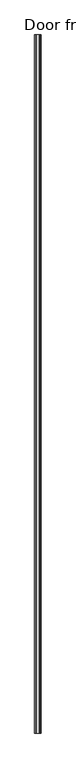
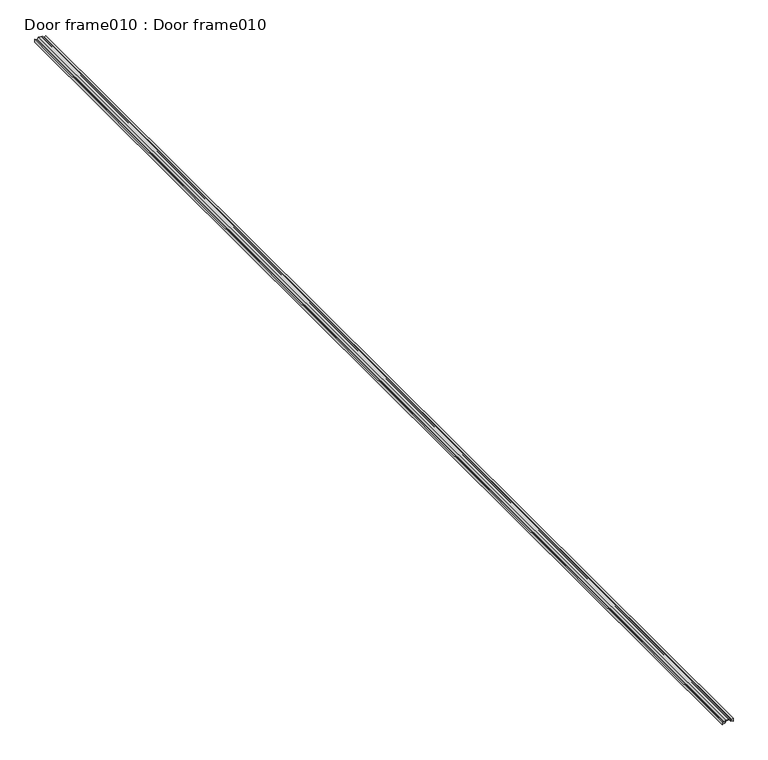
"""IFC4 building model written with IfcOpenShell, lengths in millimetres: proxy geometry, Door frame010 : Door frame010."""

from ifc_helpers import new_model, si_unit, frame, origin, place, context, project, spatial, polyline, outline, extrude, source, transform, mapped, element, save


def door_frame010_door_frame010_dc68b2cc(model_context):
    return source(origin(), model_context, "Body", "SweptSolid", [
        extrude(outline(polyline([(36662.6580816, 15538.4954576), (36662.6580816, 15540.1419606), (36665.8580816, 15542.3826247), (36665.8580816, 15547.7313685), (36662.6580816, 15549.9720326), (36662.6580816, 15551.6185356), (36661.1287449, 15554.2674246), (36665.9874184, 15554.2674246), (36664.4580816, 15551.6185356), (36664.4580816, 15550.6648984), (36667.4580816, 15548.5642757), (36667.4580816, 15541.5497174), (36664.4580816, 15539.4490948), (36664.4580816, 15538.4954576), (36666.0170308, 15535.7952784), (36661.0991325, 15535.7952784), (36662.6580816, 15538.4954576)])), frame((0.0, -1052.8906567, 0.0), z_axis=(0.0, 1.0, 0.0), x_axis=(0.0, 0.0, 1.0)), (0.0, 0.0, 1.0), 1999.85),
    ])


if __name__ == "__main__":
    model = new_model("IFC4")
    model_context = context("Model", 3, world=origin())
    ifc_project = project(units=[si_unit("LENGTHUNIT", "METRE", prefix="MILLI")], contexts=[model_context])
    site = spatial("IfcSite", under=ifc_project)
    building = spatial("IfcBuilding", under=site)
    placement = place(None, origin())
    door_frame010_door_frame010_shape = door_frame010_door_frame010_dc68b2cc(model_context)
    element("IfcBuildingElementProxy", 1, Name="Door frame010 : Door frame010", ObjectType="Door frame010 : Door frame010", at=placement, inside=building, context=model_context, shape_type="MappedRepresentation", body=[
        mapped(door_frame010_door_frame010_shape, transform((0.0, 0.0, 0.0), x_axis=(1.0, 0.0, 0.0), y_axis=(0.0, 1.0, 0.0), z_axis=(0.0, 0.0, 1.0))),
    ])
    save(model, "model.ifc")

# Revit data of these elements
# Type "Door frame010 : Door frame010"
#   NameOverride = "Door frame010"
# Element 1 (IfcBuildingElementProxy, "Door frame010 : Door frame010")
#   Materials on its faces: "FLEETWOOD SERIES T-3200 SINGLE SWING DOOR FRAME"
# Materials
#   "FLEETWOOD SERIES T-3200 SINGLE SWING DOOR FRAME": class "Unassigned", colour RGB 128 128 128, transparency 0, Cost = 0
